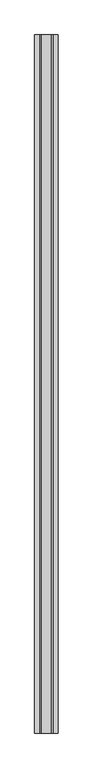
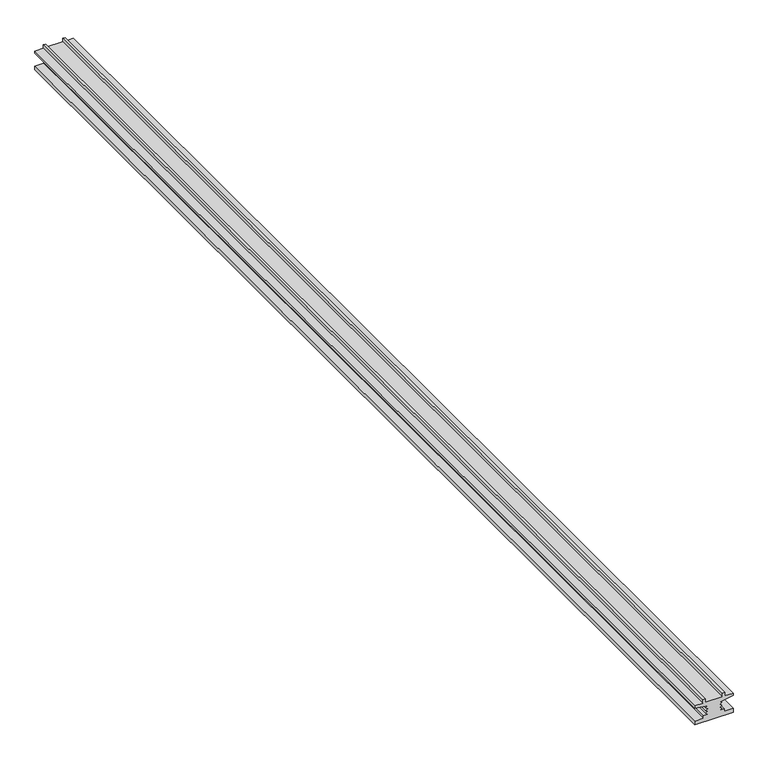
"""IFC4 building model written with IfcOpenShell, lengths in millimetres: proxy geometry, Bison pedestal1:Bison pedestal004:295339 : Bison pedestal1:Bison pedestal004:295339."""

import ifcopenshell
import ifcopenshell.guid

model = None  # the IFC model being written
_history = None  # IfcOwnerHistory: only IFC2X3 demands one
_inside = {}  # id of a spatial element -> (the spatial element, [elements in it])
_under = {}  # id of a project, library or spatial element -> (it, [spatial elements below it])
_declared = {}  # id of a project -> (the project, [libraries it declares])
_typed = {}  # id of a type object -> (the type object, [elements of that type])
_made_of = {}  # id of a material, layer set ... -> (it, [elements and type objects made of it])


def new_model(schema):
    """Start an empty IFC model of exactly this schema.

    Asked for "IFC4X3", IfcOpenShell would pick the latest addendum, in which some entities
    have other attributes; the version numbers below select the first issue.
    IFC2X3 requires an IfcOwnerHistory on every rooted entity: one is made here for all.
    """
    global model, _history
    if schema == "IFC4X3":
        model = ifcopenshell.file(schema_version=(4, 3, 0, 0))
    else:
        model = ifcopenshell.file(schema=schema)
    _inside.clear()
    _under.clear()
    _declared.clear()
    _typed.clear()
    _made_of.clear()
    _history = None
    if model.schema == "IFC2X3":
        org = make("IfcOrganization", Name="unknown")
        user = make(
            "IfcPersonAndOrganization",
            ThePerson=make("IfcPerson", FamilyName="unknown"),
            TheOrganization=org,
        )
        app = make(
            "IfcApplication",
            ApplicationDeveloper=org,
            Version="unknown",
            ApplicationFullName="unknown",
            ApplicationIdentifier="unknown",
        )
        _history = make(
            "IfcOwnerHistory",
            OwningUser=user,
            OwningApplication=app,
            ChangeAction="ADDED",
            CreationDate=0,
        )
    return model


def make(cls, **values):
    """One entity of the class cls with the attributes given. An attribute that is None is left unset."""
    return model.create_entity(
        cls, **{name: value for name, value in values.items() if value is not None}
    )


def rooted(cls, **values):
    """An entity with a GlobalId (a new one), such as an element, a storey or a relation."""
    return make(cls, GlobalId=ifcopenshell.guid.new(), OwnerHistory=_history, **values)


def si_unit(unit_type, name, prefix=None):
    """IfcSIUnit, for example si_unit("LENGTHUNIT", "METRE", prefix="MILLI")."""
    return make("IfcSIUnit", UnitType=unit_type, Prefix=prefix, Name=name)


def assignment(units):
    """IfcUnitAssignment: the units of a project."""
    return None if units is None else make("IfcUnitAssignment", Units=units)


def point(xyz):
    """IfcCartesianPoint."""
    return None if xyz is None else make("IfcCartesianPoint", Coordinates=xyz)


def direction(xyz):
    """IfcDirection."""
    return None if xyz is None else make("IfcDirection", DirectionRatios=xyz)


def frame(location, z_axis=None, x_axis=None):
    """IfcAxis2Placement3D, a coordinate frame: its origin and axes. An axis left out is left unset."""
    return make(
        "IfcAxis2Placement3D",
        Location=point(location),
        Axis=direction(z_axis),
        RefDirection=direction(x_axis),
    )


def origin():
    """The frame at (0, 0, 0) with its axes left unset."""
    return frame((0.0, 0.0, 0.0))


def place(relative_to, where):
    """IfcLocalPlacement: puts the frame where relative to a parent placement (None: the world)."""
    return make(
        "IfcLocalPlacement", PlacementRelTo=relative_to, RelativePlacement=where
    )


def context(
    kind, dimensions, precision=None, world=None, true_north=None, identifier=None
):
    """IfcGeometricRepresentationContext, for example the 3D "Model" context."""
    return make(
        "IfcGeometricRepresentationContext",
        ContextIdentifier=identifier,
        ContextType=kind,
        CoordinateSpaceDimension=dimensions,
        Precision=precision,
        WorldCoordinateSystem=world,
        TrueNorth=true_north,
    )


def project(units=None, contexts=None):
    """IfcProject with its units and contexts."""
    return rooted(
        "IfcProject",
        Name="project",
        RepresentationContexts=contexts,
        UnitsInContext=assignment(units),
    )


def spatial(cls, under=None, at=None, **own):
    """A site, building, storey or space (cls), placed at a placement, below another one or the project."""
    s = rooted(cls, ObjectPlacement=at, **own)
    if under is not None:
        _under.setdefault(under.id(), (under, []))[1].append(s)
    return s


def polyline(points):
    """IfcPolyline through the points."""
    return make("IfcPolyline", Points=[point(p) for p in points])


def outline(outer, holes=None, kind="AREA"):
    """IfcArbitraryClosedProfileDef: a profile drawn as a closed curve; with holes, ...WithVoids."""
    if holes is None:
        return make("IfcArbitraryClosedProfileDef", ProfileType=kind, OuterCurve=outer)
    return make(
        "IfcArbitraryProfileDefWithVoids",
        ProfileType=kind,
        OuterCurve=outer,
        InnerCurves=holes,
    )


def extrude(swept, where, along, depth):
    """IfcExtrudedAreaSolid: the profile swept, set in the frame where, extruded along a direction by depth."""
    return make(
        "IfcExtrudedAreaSolid",
        SweptArea=swept,
        Position=where,
        ExtrudedDirection=direction(along),
        Depth=depth,
    )


def shape(context_of_items, identifier, shape_type, items):
    """IfcShapeRepresentation: the items that make up one representation, for example the "Body"."""
    return make(
        "IfcShapeRepresentation",
        ContextOfItems=context_of_items,
        RepresentationIdentifier=identifier,
        RepresentationType=shape_type,
        Items=items,
    )


def source(mapping_origin, context_of_items, identifier, shape_type, items):
    """IfcRepresentationMap: a shape defined once, which mapped items show again and again."""
    return make(
        "IfcRepresentationMap",
        MappingOrigin=mapping_origin,
        MappedRepresentation=shape(context_of_items, identifier, shape_type, items),
    )


def transform(
    local_origin,
    x_axis=None,
    y_axis=None,
    z_axis=None,
    scale=None,
    scale2=None,
    scale3=None,
    uniform=True,
):
    """IfcCartesianTransformationOperator3D, or its non-uniform kind. x_axis, y_axis, z_axis: its Axis1, 2, 3."""
    if uniform:
        return make(
            "IfcCartesianTransformationOperator3D",
            Axis1=direction(x_axis),
            Axis2=direction(y_axis),
            LocalOrigin=point(local_origin),
            Scale=scale,
            Axis3=direction(z_axis),
        )
    return make(
        "IfcCartesianTransformationOperator3DnonUniform",
        Axis1=direction(x_axis),
        Axis2=direction(y_axis),
        LocalOrigin=point(local_origin),
        Scale=scale,
        Axis3=direction(z_axis),
        Scale2=scale2,
        Scale3=scale3,
    )


def mapped(mapping_source, mapping_target):
    """IfcMappedItem: shows the shape of a source again, moved by a transform."""
    return make(
        "IfcMappedItem", MappingSource=mapping_source, MappingTarget=mapping_target
    )


def made_of(thing, what):
    """Note that an element or type object is made of a material, layer set ...; save() writes the relation."""
    if what is not None:
        _made_of.setdefault(what.id(), (what, []))[1].append(thing)
    return thing


def element(
    cls,
    number,
    at=None,
    inside=None,
    cuts=None,
    type_object=None,
    material=None,
    context=None,
    identifier="Body",
    shape_type=None,
    held_by="IfcProductDefinitionShape",
    body=None,
    shapes=None,
    **own,
):
    """One element of the class cls, such as IfcWall. Its Tag is "e" and its number.

    at: its placement. inside: the storey or other place that contains it. cuts: it is an
    opening in that element (IfcRelVoidsElement). A single representation is given by context,
    identifier, shape_type and body (its items); several are given by shapes. held_by: the class
    of the entity that holds the representations. save() writes the other relations.
    """
    e = rooted(cls, Tag="e%d" % number, ObjectPlacement=at, **own)
    if body is not None:
        shapes = [shape(context, identifier, shape_type, body)]
    if shapes is not None:
        e.Representation = make(held_by, Representations=shapes)
    if inside is not None:
        _inside.setdefault(inside.id(), (inside, []))[1].append(e)
    if cuts is not None:
        rooted(
            "IfcRelVoidsElement", RelatingBuildingElement=cuts, RelatedOpeningElement=e
        )
    if type_object is not None:
        _typed.setdefault(type_object.id(), (type_object, []))[1].append(e)
    return made_of(e, material)


def aggregate(whole, parts):
    """IfcRelAggregates: a whole, such as a stair, and the parts it consists of."""
    return rooted("IfcRelAggregates", RelatingObject=whole, RelatedObjects=parts)


def save(model, path):
    """Write the relations noted so far, then the file.

    IfcRelAggregates (storeys below a building ...), IfcRelContainedInSpatialStructure (elements
    in a storey), IfcRelDefinesByType, IfcRelAssociatesMaterial and IfcRelDeclares: one each for
    every whole, place, type object, material and project.
    """
    for whole, parts in _under.values():
        aggregate(whole, parts)
    for where, things in _inside.values():
        rooted(
            "IfcRelContainedInSpatialStructure",
            RelatedElements=things,
            RelatingStructure=where,
        )
    for kind, things in _typed.values():
        rooted("IfcRelDefinesByType", RelatedObjects=things, RelatingType=kind)
    for what, things in _made_of.values():
        rooted("IfcRelAssociatesMaterial", RelatedObjects=things, RelatingMaterial=what)
    for by, libraries in _declared.values():
        rooted("IfcRelDeclares", RelatingContext=by, RelatedDefinitions=libraries)
    model.write(path)


def generic_models_7c9c526c(model_context):
    return source(origin(), model_context, "Body", "SweptSolid", [
        extrude(outline(polyline([(36480.0342739, 1966.5338754), (36480.0342739, 2033.9545554), (36486.734375, 2034.0191178), (36486.734375, 2018.5996842), (36491.2120625, 2018.5996842), (36491.2120625, 2010.5086197), (36494.1534687, 2014.0393814), (36496.7296406, 2010.7293228), (36499.4503437, 2014.2598404), (36502.0245625, 2010.8762955), (36504.5577656, 2014.4510025), (36507.1046406, 2011.2344498), (36510.9913594, 2034.0191178), (36515.1456562, 2034.0191178), (36515.1456562, 2019.2759537), (36521.3116719, 2019.2759537), (36521.3116719, 2015.3892349), (36515.1456562, 2015.3892349), (36515.1456562, 1985.0991959), (36521.3116719, 1985.0991959), (36521.3116719, 1981.2124771), (36515.1456562, 1981.2124771), (36515.1456562, 1966.4693131), (36510.9913594, 1966.4693131), (36507.1046406, 1989.253981), (36504.5577656, 1986.0374283), (36502.0245625, 1989.6121353), (36499.4503437, 1986.2285904), (36496.7296406, 1989.759108), (36494.1534687, 1986.4490494), (36491.2120625, 1989.9798111), (36491.2120625, 1981.8887467), (36486.734375, 1981.8887467), (36486.734375, 1966.4693131), (36480.0342739, 1966.5338754)])), frame((0.0, 1276.4895464, 0.0), z_axis=(0.0, 1.0, 0.0), x_axis=(0.0, 0.0, 1.0)), (0.0, 0.0, 1.0), 2000.0),
    ])


if __name__ == "__main__":
    model = new_model("IFC4")
    model_context = context("Model", 3, world=origin())
    ifc_project = project(units=[si_unit("LENGTHUNIT", "METRE", prefix="MILLI")], contexts=[model_context])
    site = spatial("IfcSite", under=ifc_project)
    building = spatial("IfcBuilding", under=site)
    placement = place(None, origin())
    generic_models_shape = generic_models_7c9c526c(model_context)
    element("IfcBuildingElementProxy", 1, Name="Bison pedestal1:Bison pedestal004:295339 : Bison pedestal1:Bison pedestal004:295339", ObjectType="Bison pedestal1:Bison pedestal004:295339 : Bison pedestal1:Bison pedestal004:295339", at=placement, inside=building, context=model_context, shape_type="MappedRepresentation", body=[
        mapped(generic_models_shape, transform((0.0, 0.0, 0.0), x_axis=(1.0, 0.0, 0.0), y_axis=(0.0, 1.0, 0.0), z_axis=(0.0, 0.0, 1.0))),
    ])
    save(model, "model.ifc")

# Revit data of these elements
# Type "Bison pedestal1:Bison pedestal004:295339 : Bison pedestal1:Bison pedestal004:295339"
#   NameOverride = "Bison pedestal1:Bison pedestal004:295339"
#   ObjectTypeOverride = "Bison pedestal1:Bison pedestal004"
#   Reference = "Bison pedestal004"
#   Category = "Generic Models"
#   Tag = "295339"
# Element 1 (IfcBuildingElementProxy, "Bison pedestal1:Bison pedestal004:295339 : Bison pedestal1:Bison pedestal004:295339")
#   Materials on its faces: "BUZON PEDESTAL"
# Materials
#   "BUZON PEDESTAL": class "Unassigned", colour RGB 66 66 66, transparency 0
